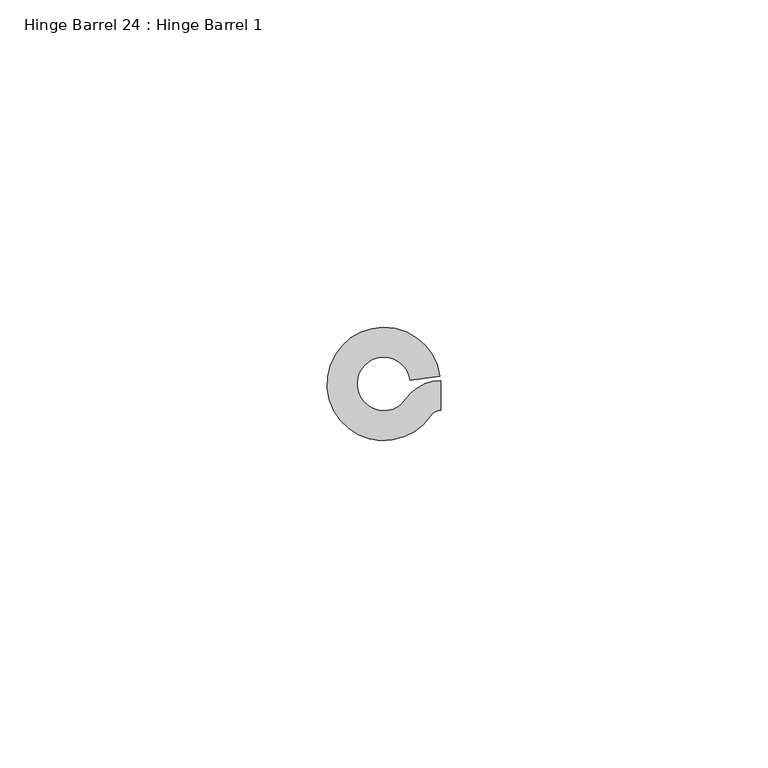
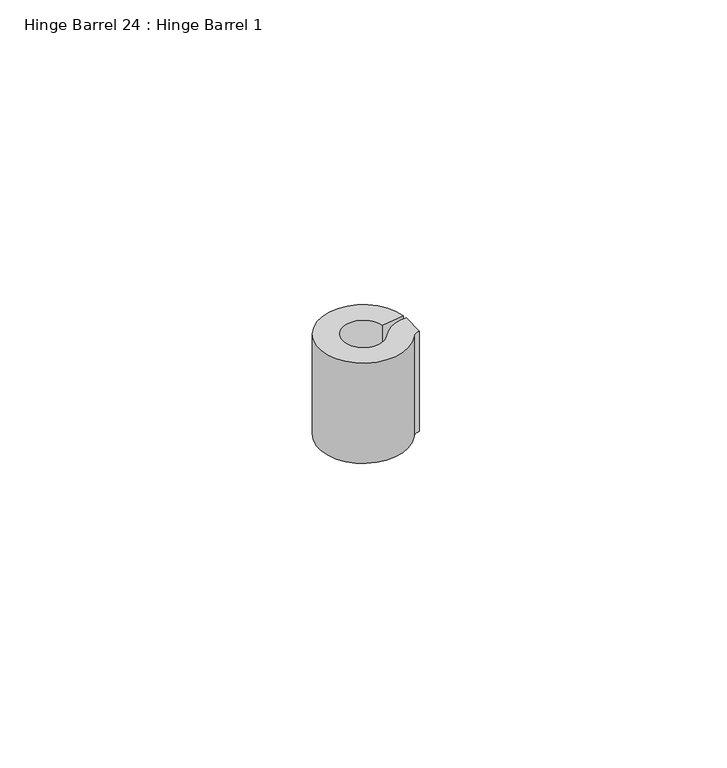
"""IFC4 building model written with IfcOpenShell, lengths in millimetres: proxy geometry, Hinge Barrel 24 : Hinge Barrel 1."""

from ifc_helpers import new_model, si_unit, point, frame, frame_2d, origin, place, context, project, spatial, polyline, circle_curve, trimmed, segment, composite_curve, outline, extrude, source, transform, mapped, element, save


def hinge_barrel_24_hinge_barrel_1_d5905ef5(model_context):
    return source(origin(), model_context, "Body", "SweptSolid", [
        extrude(outline(composite_curve([segment(trimmed(circle_curve(frame_2d((587327.8245257, -533990.5568067)), 6.4044851), [point((587322.5194669, -533986.9688017))], [point((587327.8245257, -533984.1523216))], False, "CARTESIAN"), True, "CONTINUOUS"), segment(polyline([(587327.8245257, -533984.1523216), (587327.8245257, -533988.7163841)]), True, "CONTINUOUS"), segment(trimmed(circle_curve(frame_2d((587327.8245257, -533990.5568067)), 1.8404226), [point((587327.8245257, -533988.7163841))], [point((587326.3000393, -533989.5257409))], True, "CARTESIAN"), True, "CONTINUOUS"), segment(trimmed(circle_curve(frame_2d((587319.1320739, -533984.6777841)), 8.6534625), [point((587326.3000393, -533989.5257409))], [point((587327.7022899, -533983.4803654))], False, "CARTESIAN"), True, "CONTINUOUS"), segment(polyline([(587327.7022899, -533983.4803654), (587323.1821338, -533984.1119153)]), True, "CONTINUOUS"), segment(trimmed(circle_curve(frame_2d((587319.1320739, -533984.6777841)), 4.0894), [point((587323.1821338, -533984.1119153))], [point((587322.5194669, -533986.9688017))], True, "CARTESIAN"), True, "CONTINUOUS")], self_intersect=False)), frame((0.0, 0.0, 2063.75), z_axis=(0.0, 0.0, 1.0), x_axis=(1.0, 0.0, 0.0)), (0.0, 0.0, 1.0), 20.8359375),
    ])


if __name__ == "__main__":
    model = new_model("IFC4")
    model_context = context("Model", 3, world=origin())
    ifc_project = project(units=[si_unit("LENGTHUNIT", "METRE", prefix="MILLI")], contexts=[model_context])
    site = spatial("IfcSite", under=ifc_project)
    building = spatial("IfcBuilding", under=site)
    placement = place(None, origin())
    hinge_barrel_24_hinge_barrel_1_shape = hinge_barrel_24_hinge_barrel_1_d5905ef5(model_context)
    element("IfcBuildingElementProxy", 1, Name="Hinge Barrel 24 : Hinge Barrel 1", ObjectType="Hinge Barrel 24 : Hinge Barrel 1", at=placement, inside=building, context=model_context, shape_type="MappedRepresentation", body=[
        mapped(hinge_barrel_24_hinge_barrel_1_shape, transform((0.0, 0.0, 0.0), x_axis=(1.0, 0.0, 0.0), y_axis=(0.0, 1.0, 0.0), z_axis=(0.0, 0.0, 1.0))),
    ])
    save(model, "model.ifc")

# Revit data of these elements
# Element 1 (IfcBuildingElementProxy, "Hinge Barrel 24 : Hinge Barrel 1")
#   Materials on its faces: "6\"X6\" WELD-ON STL BUTT HINGE"
# Materials
#   "6\"X6\" WELD-ON STL BUTT HINGE": class "Metal", colour RGB 189 187 185, transparency 0, Description = "Carbon steel", Cost = 0
